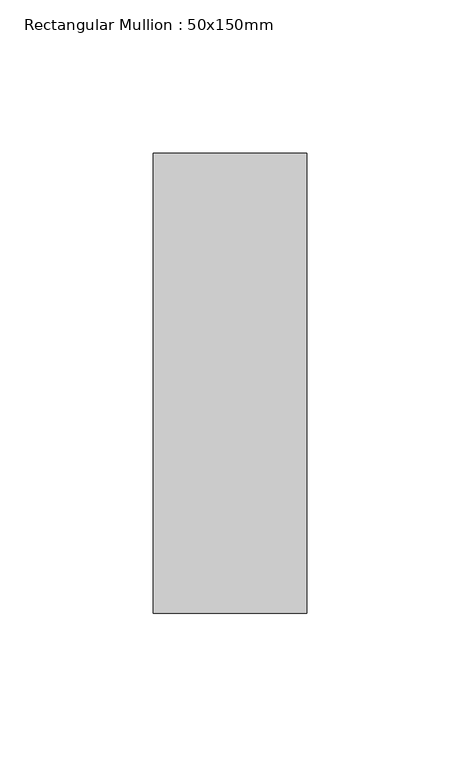
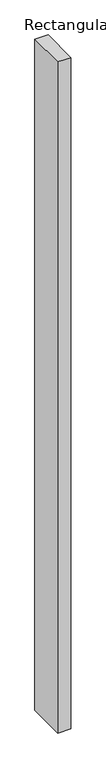
"""IFC4 building model written with IfcOpenShell, lengths in millimetres: member geometry, Rectangular Mullion : 50x150mm."""

import ifcopenshell
import ifcopenshell.guid

model = None  # the IFC model being written
_history = None  # IfcOwnerHistory: only IFC2X3 demands one
_inside = {}  # id of a spatial element -> (the spatial element, [elements in it])
_under = {}  # id of a project, library or spatial element -> (it, [spatial elements below it])
_declared = {}  # id of a project -> (the project, [libraries it declares])
_typed = {}  # id of a type object -> (the type object, [elements of that type])
_made_of = {}  # id of a material, layer set ... -> (it, [elements and type objects made of it])


def new_model(schema):
    """Start an empty IFC model of exactly this schema.

    Asked for "IFC4X3", IfcOpenShell would pick the latest addendum, in which some entities
    have other attributes; the version numbers below select the first issue.
    IFC2X3 requires an IfcOwnerHistory on every rooted entity: one is made here for all.
    """
    global model, _history
    if schema == "IFC4X3":
        model = ifcopenshell.file(schema_version=(4, 3, 0, 0))
    else:
        model = ifcopenshell.file(schema=schema)
    _inside.clear()
    _under.clear()
    _declared.clear()
    _typed.clear()
    _made_of.clear()
    _history = None
    if model.schema == "IFC2X3":
        org = make("IfcOrganization", Name="unknown")
        user = make(
            "IfcPersonAndOrganization",
            ThePerson=make("IfcPerson", FamilyName="unknown"),
            TheOrganization=org,
        )
        app = make(
            "IfcApplication",
            ApplicationDeveloper=org,
            Version="unknown",
            ApplicationFullName="unknown",
            ApplicationIdentifier="unknown",
        )
        _history = make(
            "IfcOwnerHistory",
            OwningUser=user,
            OwningApplication=app,
            ChangeAction="ADDED",
            CreationDate=0,
        )
    return model


def make(cls, **values):
    """One entity of the class cls with the attributes given. An attribute that is None is left unset."""
    return model.create_entity(
        cls, **{name: value for name, value in values.items() if value is not None}
    )


def rooted(cls, **values):
    """An entity with a GlobalId (a new one), such as an element, a storey or a relation."""
    return make(cls, GlobalId=ifcopenshell.guid.new(), OwnerHistory=_history, **values)


def si_unit(unit_type, name, prefix=None):
    """IfcSIUnit, for example si_unit("LENGTHUNIT", "METRE", prefix="MILLI")."""
    return make("IfcSIUnit", UnitType=unit_type, Prefix=prefix, Name=name)


def assignment(units):
    """IfcUnitAssignment: the units of a project."""
    return None if units is None else make("IfcUnitAssignment", Units=units)


def point(xyz):
    """IfcCartesianPoint."""
    return None if xyz is None else make("IfcCartesianPoint", Coordinates=xyz)


def direction(xyz):
    """IfcDirection."""
    return None if xyz is None else make("IfcDirection", DirectionRatios=xyz)


def frame(location, z_axis=None, x_axis=None):
    """IfcAxis2Placement3D, a coordinate frame: its origin and axes. An axis left out is left unset."""
    return make(
        "IfcAxis2Placement3D",
        Location=point(location),
        Axis=direction(z_axis),
        RefDirection=direction(x_axis),
    )


def origin():
    """The frame at (0, 0, 0) with its axes left unset."""
    return frame((0.0, 0.0, 0.0))


def place(relative_to, where):
    """IfcLocalPlacement: puts the frame where relative to a parent placement (None: the world)."""
    return make(
        "IfcLocalPlacement", PlacementRelTo=relative_to, RelativePlacement=where
    )


def context(
    kind, dimensions, precision=None, world=None, true_north=None, identifier=None
):
    """IfcGeometricRepresentationContext, for example the 3D "Model" context."""
    return make(
        "IfcGeometricRepresentationContext",
        ContextIdentifier=identifier,
        ContextType=kind,
        CoordinateSpaceDimension=dimensions,
        Precision=precision,
        WorldCoordinateSystem=world,
        TrueNorth=true_north,
    )


def project(units=None, contexts=None):
    """IfcProject with its units and contexts."""
    return rooted(
        "IfcProject",
        Name="project",
        RepresentationContexts=contexts,
        UnitsInContext=assignment(units),
    )


def spatial(cls, under=None, at=None, **own):
    """A site, building, storey or space (cls), placed at a placement, below another one or the project."""
    s = rooted(cls, ObjectPlacement=at, **own)
    if under is not None:
        _under.setdefault(under.id(), (under, []))[1].append(s)
    return s


def polyline(points):
    """IfcPolyline through the points."""
    return make("IfcPolyline", Points=[point(p) for p in points])


def outline(outer, holes=None, kind="AREA"):
    """IfcArbitraryClosedProfileDef: a profile drawn as a closed curve; with holes, ...WithVoids."""
    if holes is None:
        return make("IfcArbitraryClosedProfileDef", ProfileType=kind, OuterCurve=outer)
    return make(
        "IfcArbitraryProfileDefWithVoids",
        ProfileType=kind,
        OuterCurve=outer,
        InnerCurves=holes,
    )


def extrude(swept, where, along, depth):
    """IfcExtrudedAreaSolid: the profile swept, set in the frame where, extruded along a direction by depth."""
    return make(
        "IfcExtrudedAreaSolid",
        SweptArea=swept,
        Position=where,
        ExtrudedDirection=direction(along),
        Depth=depth,
    )


def shape(context_of_items, identifier, shape_type, items):
    """IfcShapeRepresentation: the items that make up one representation, for example the "Body"."""
    return make(
        "IfcShapeRepresentation",
        ContextOfItems=context_of_items,
        RepresentationIdentifier=identifier,
        RepresentationType=shape_type,
        Items=items,
    )


def source(mapping_origin, context_of_items, identifier, shape_type, items):
    """IfcRepresentationMap: a shape defined once, which mapped items show again and again."""
    return make(
        "IfcRepresentationMap",
        MappingOrigin=mapping_origin,
        MappedRepresentation=shape(context_of_items, identifier, shape_type, items),
    )


def transform(
    local_origin,
    x_axis=None,
    y_axis=None,
    z_axis=None,
    scale=None,
    scale2=None,
    scale3=None,
    uniform=True,
):
    """IfcCartesianTransformationOperator3D, or its non-uniform kind. x_axis, y_axis, z_axis: its Axis1, 2, 3."""
    if uniform:
        return make(
            "IfcCartesianTransformationOperator3D",
            Axis1=direction(x_axis),
            Axis2=direction(y_axis),
            LocalOrigin=point(local_origin),
            Scale=scale,
            Axis3=direction(z_axis),
        )
    return make(
        "IfcCartesianTransformationOperator3DnonUniform",
        Axis1=direction(x_axis),
        Axis2=direction(y_axis),
        LocalOrigin=point(local_origin),
        Scale=scale,
        Axis3=direction(z_axis),
        Scale2=scale2,
        Scale3=scale3,
    )


def mapped(mapping_source, mapping_target):
    """IfcMappedItem: shows the shape of a source again, moved by a transform."""
    return make(
        "IfcMappedItem", MappingSource=mapping_source, MappingTarget=mapping_target
    )


def made_of(thing, what):
    """Note that an element or type object is made of a material, layer set ...; save() writes the relation."""
    if what is not None:
        _made_of.setdefault(what.id(), (what, []))[1].append(thing)
    return thing


def element(
    cls,
    number,
    at=None,
    inside=None,
    cuts=None,
    type_object=None,
    material=None,
    context=None,
    identifier="Body",
    shape_type=None,
    held_by="IfcProductDefinitionShape",
    body=None,
    shapes=None,
    **own,
):
    """One element of the class cls, such as IfcWall. Its Tag is "e" and its number.

    at: its placement. inside: the storey or other place that contains it. cuts: it is an
    opening in that element (IfcRelVoidsElement). A single representation is given by context,
    identifier, shape_type and body (its items); several are given by shapes. held_by: the class
    of the entity that holds the representations. save() writes the other relations.
    """
    e = rooted(cls, Tag="e%d" % number, ObjectPlacement=at, **own)
    if body is not None:
        shapes = [shape(context, identifier, shape_type, body)]
    if shapes is not None:
        e.Representation = make(held_by, Representations=shapes)
    if inside is not None:
        _inside.setdefault(inside.id(), (inside, []))[1].append(e)
    if cuts is not None:
        rooted(
            "IfcRelVoidsElement", RelatingBuildingElement=cuts, RelatedOpeningElement=e
        )
    if type_object is not None:
        _typed.setdefault(type_object.id(), (type_object, []))[1].append(e)
    return made_of(e, material)


def aggregate(whole, parts):
    """IfcRelAggregates: a whole, such as a stair, and the parts it consists of."""
    return rooted("IfcRelAggregates", RelatingObject=whole, RelatedObjects=parts)


def save(model, path):
    """Write the relations noted so far, then the file.

    IfcRelAggregates (storeys below a building ...), IfcRelContainedInSpatialStructure (elements
    in a storey), IfcRelDefinesByType, IfcRelAssociatesMaterial and IfcRelDeclares: one each for
    every whole, place, type object, material and project.
    """
    for whole, parts in _under.values():
        aggregate(whole, parts)
    for where, things in _inside.values():
        rooted(
            "IfcRelContainedInSpatialStructure",
            RelatedElements=things,
            RelatingStructure=where,
        )
    for kind, things in _typed.values():
        rooted("IfcRelDefinesByType", RelatedObjects=things, RelatingType=kind)
    for what, things in _made_of.values():
        rooted("IfcRelAssociatesMaterial", RelatedObjects=things, RelatingMaterial=what)
    for by, libraries in _declared.values():
        rooted("IfcRelDeclares", RelatingContext=by, RelatedDefinitions=libraries)
    model.write(path)


def rectangular_mullion_50x150mm_cf0a7a0a(model_context):
    return source(origin(), model_context, "Body", "SweptSolid", [
        extrude(outline(polyline([(25.0, 75.0), (25.0, -75.0), (-25.0, -75.0), (-25.0, 75.0), (25.0, 75.0)])), frame((0.0, 0.0, -2700.0), z_axis=(0.0, 0.0, 1.0), x_axis=(1.0, 0.0, 0.0)), (0.0, 0.0, 1.0), 2700.0),
    ])


if __name__ == "__main__":
    model = new_model("IFC4")
    model_context = context("Model", 3, world=origin())
    ifc_project = project(units=[si_unit("LENGTHUNIT", "METRE", prefix="MILLI")], contexts=[model_context])
    site = spatial("IfcSite", under=ifc_project)
    building = spatial("IfcBuilding", under=site)
    placement = place(None, origin())
    rectangular_mullion_50x150mm_shape = rectangular_mullion_50x150mm_cf0a7a0a(model_context)
    element("IfcMember", 1, ObjectType="Rectangular Mullion : 50x150mm", at=placement, inside=building, context=model_context, shape_type="MappedRepresentation", body=[
        mapped(rectangular_mullion_50x150mm_shape, transform((0.0, 0.0, 0.0), x_axis=(1.0, 0.0, 0.0), y_axis=(0.0, 1.0, 0.0), z_axis=(0.0, 0.0, 1.0))),
    ])
    save(model, "model.ifc")

# Revit data of these elements
# Type "Rectangular Mullion : 50x150mm"
#   Keynote = "H11"
#   built-in parameter 1007304 = 0.492126 (stored number, unit not read)
#   built-in parameter 1007301 = 0.082021 (stored number, unit not read)
#   built-in parameter 1007300 = 0.082021 (stored number, unit not read)
# Element 1 (IfcMember, "Rectangular Mullion : 50x150mm")
#   Materials on its faces: "Aluminium"
# Materials
#   "Aluminium": class "Metal", colour RGB 247 247 247, transparency 0, Description = "Aluminium 6061", Cost = 0
